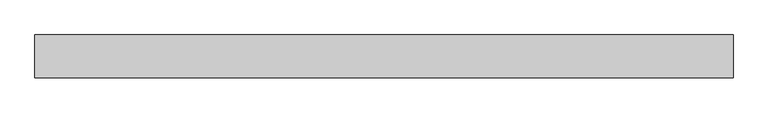
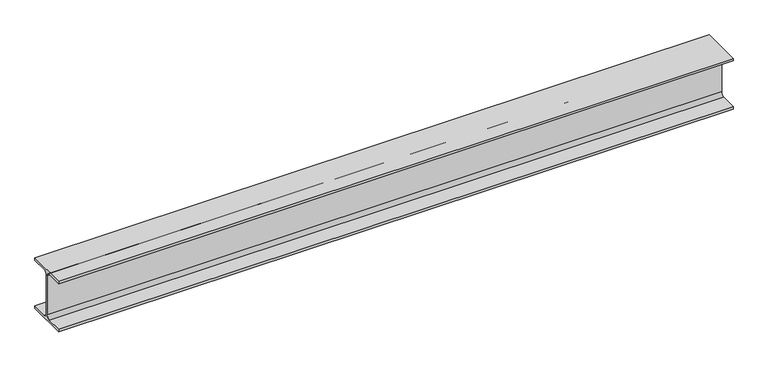
"""IFC4 building model written with IfcOpenShell, lengths in millimetres: beam geometry, 0912_Steel Framing_H-KSD3502 : H_SB_ASB_H-194x150x6x9."""

from ifc_helpers import new_model, si_unit, point, frame, frame_2d, origin, place, context, project, spatial, polyline, circle_curve, trimmed, segment, composite_curve, outline, extrude, source, transform, mapped, element, save


def beam_1fcf74dc(model_context):
    return source(origin(), model_context, "Body", "SweptSolid", [
        extrude(outline(composite_curve([segment(polyline([(-75.0, -88.0), (-16.0, -88.0)]), True, "CONTINUOUS"), segment(trimmed(circle_curve(frame_2d((-16.0, -75.0)), 13.0), [point((-16.0, -88.0))], [point((-3.0, -75.0))], True, "CARTESIAN"), True, "CONTINUOUS"), segment(polyline([(-3.0, -75.0), (-3.0, 75.0)]), True, "CONTINUOUS"), segment(trimmed(circle_curve(frame_2d((-16.0, 75.0)), 13.0), [point((-3.0, 75.0))], [point((-16.0, 88.0))], True, "CARTESIAN"), True, "CONTINUOUS"), segment(polyline([(-16.0, 88.0), (-75.0, 88.0), (-75.0, 97.0), (75.0, 97.0), (75.0, 88.0), (16.0, 88.0)]), True, "CONTINUOUS"), segment(trimmed(circle_curve(frame_2d((16.0, 75.0)), 13.0), [point((16.0, 88.0))], [point((3.0, 75.0))], True, "CARTESIAN"), True, "CONTINUOUS"), segment(polyline([(3.0, 75.0), (3.0, -75.0)]), True, "CONTINUOUS"), segment(trimmed(circle_curve(frame_2d((16.0, -75.0)), 13.0), [point((3.0, -75.0))], [point((16.0, -88.0))], True, "CARTESIAN"), True, "CONTINUOUS"), segment(polyline([(16.0, -88.0), (75.0, -88.0), (75.0, -97.0), (-75.0, -97.0), (-75.0, -88.0)]), True, "CONTINUOUS")], self_intersect=False)), frame((-1200.0, 0.0, 0.0), z_axis=(1.0, 0.0, 0.0), x_axis=(0.0, 1.0, 0.0)), (0.0, 0.0, 1.0), 2453.1701073),
    ])


if __name__ == "__main__":
    model = new_model("IFC4")
    model_context = context("Model", 3, world=origin())
    ifc_project = project(units=[si_unit("LENGTHUNIT", "METRE", prefix="MILLI")], contexts=[model_context])
    site = spatial("IfcSite", under=ifc_project)
    building = spatial("IfcBuilding", under=site)
    placement = place(None, origin())
    beam_shape = beam_1fcf74dc(model_context)
    element("IfcBeam", 1, ObjectType="0912_Steel Framing_H-KSD3502 : H_SB_ASB_H-194x150x6x9", at=placement, inside=building, context=model_context, shape_type="MappedRepresentation", body=[
        mapped(beam_shape, transform((0.0, 0.0, 0.0), x_axis=(1.0, 0.0, 0.0), y_axis=(0.0, 1.0, 0.0), z_axis=(0.0, 0.0, 1.0))),
    ])
    save(model, "model.ifc")

# Revit data of these elements
# Type "0912_Steel Framing_H-KSD3502 : H_SB_ASB_H-194x150x6x9"
#   H_WM Code_1 = "S01AA002-00001 | Main Steel Structure Fabrication Work | Shelter/Building | Medium Steel - Standard (90KG/M>Weight≥30KG/M) | Material: (   )"
#   H_WM Code_2 = "S03AA028-00001 | Main Steel Structure Erection Work | Shelter/Building | Medium Steel (90KG/M>Weight≥30KG/M) | Material: (   )"
#   H_WM Code_3 = "S01AA010-00001 | Main Steel Structure Fabrication Work | Shelter/Building | Steel Painting/Coating | for Non-Fireproofed Steel Surface, Surface Preparation, Primer, Second & Final Coat | Material: (   )"
#   H_Q'ty Cal Type Tag = "SB-Q2"
#   Width = 15.0 cm
#   Web Thickness = 0.6 cm
#   Web Fillet = 1.3 cm
#   Warping Constant = 43316.0 cm⁶
#   W = 0
#   Torsional Moment of Inertia = 8.622 cm⁴
#   Section Area = 39.01 cm²
#   Plastic Modulus weak axis = 104.0 cm³
#   Plastic Modulus strong axis = 309.0 cm³
#   Perimeter = 0.95 m²/m
#   Nominal Weight = 30.60 kgf/m
#   Moment of Inertia weak axis = 507.00 cm⁴
#   Moment of Inertia strong axis = 2690.00 cm⁴
#   Height = 19.4 cm
#   Flange Thickness = 0.9 cm
#   Elastic Modulus weak axis = 67.6 cm³
#   Elastic Modulus strong axis = 277.0 cm³
#   Centroid Vertical = 9.7 cm
#   Centroid Horizontal = 7.5 cm
#   Ix = 26900000
#   Length [instance default] = 1.5240 m
#   Zx = 309000
#   b = 0.1500 m
#   h = 0.1940 m
#   r = 0.0130 m
#   s = 0.0060 m
#   t = 0.0090 m
#   A = 0.003901 m²
#   Structural Material [instance default] = Steel, 45-345
#   Assembly Code = ""
# Element 1 (IfcBeam, "0912_Steel Framing_H-KSD3502 : H_SB_ASB_H-194x150x6x9")
#   Structural Material = none
# Materials
#   "Steel, 45-345": class "Metal", colour RGB 189 187 185, transparency 0, Description = "Steel 345 MPa", Cost = 0
